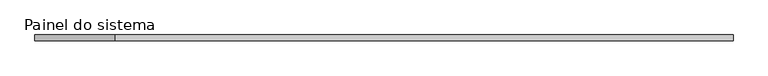
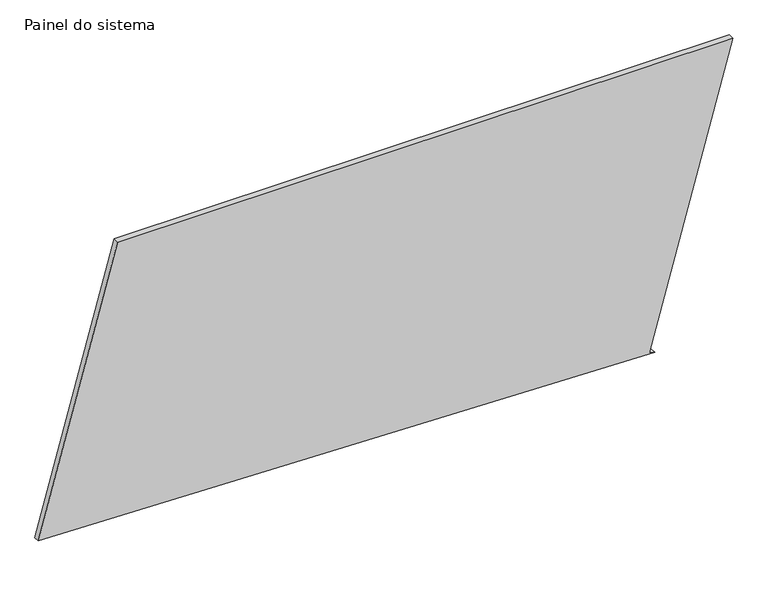
"""IFC4 building model written with IfcOpenShell, lengths in millimetres: plate geometry, Painel do sistema : Envidraçado."""

import ifcopenshell
import ifcopenshell.guid

model = None  # the IFC model being written
_history = None  # IfcOwnerHistory: only IFC2X3 demands one
_inside = {}  # id of a spatial element -> (the spatial element, [elements in it])
_under = {}  # id of a project, library or spatial element -> (it, [spatial elements below it])
_declared = {}  # id of a project -> (the project, [libraries it declares])
_typed = {}  # id of a type object -> (the type object, [elements of that type])
_made_of = {}  # id of a material, layer set ... -> (it, [elements and type objects made of it])


def new_model(schema):
    """Start an empty IFC model of exactly this schema.

    Asked for "IFC4X3", IfcOpenShell would pick the latest addendum, in which some entities
    have other attributes; the version numbers below select the first issue.
    IFC2X3 requires an IfcOwnerHistory on every rooted entity: one is made here for all.
    """
    global model, _history
    if schema == "IFC4X3":
        model = ifcopenshell.file(schema_version=(4, 3, 0, 0))
    else:
        model = ifcopenshell.file(schema=schema)
    _inside.clear()
    _under.clear()
    _declared.clear()
    _typed.clear()
    _made_of.clear()
    _history = None
    if model.schema == "IFC2X3":
        org = make("IfcOrganization", Name="unknown")
        user = make(
            "IfcPersonAndOrganization",
            ThePerson=make("IfcPerson", FamilyName="unknown"),
            TheOrganization=org,
        )
        app = make(
            "IfcApplication",
            ApplicationDeveloper=org,
            Version="unknown",
            ApplicationFullName="unknown",
            ApplicationIdentifier="unknown",
        )
        _history = make(
            "IfcOwnerHistory",
            OwningUser=user,
            OwningApplication=app,
            ChangeAction="ADDED",
            CreationDate=0,
        )
    return model


def make(cls, **values):
    """One entity of the class cls with the attributes given. An attribute that is None is left unset."""
    return model.create_entity(
        cls, **{name: value for name, value in values.items() if value is not None}
    )


def rooted(cls, **values):
    """An entity with a GlobalId (a new one), such as an element, a storey or a relation."""
    return make(cls, GlobalId=ifcopenshell.guid.new(), OwnerHistory=_history, **values)


def si_unit(unit_type, name, prefix=None):
    """IfcSIUnit, for example si_unit("LENGTHUNIT", "METRE", prefix="MILLI")."""
    return make("IfcSIUnit", UnitType=unit_type, Prefix=prefix, Name=name)


def assignment(units):
    """IfcUnitAssignment: the units of a project."""
    return None if units is None else make("IfcUnitAssignment", Units=units)


def point(xyz):
    """IfcCartesianPoint."""
    return None if xyz is None else make("IfcCartesianPoint", Coordinates=xyz)


def direction(xyz):
    """IfcDirection."""
    return None if xyz is None else make("IfcDirection", DirectionRatios=xyz)


def frame(location, z_axis=None, x_axis=None):
    """IfcAxis2Placement3D, a coordinate frame: its origin and axes. An axis left out is left unset."""
    return make(
        "IfcAxis2Placement3D",
        Location=point(location),
        Axis=direction(z_axis),
        RefDirection=direction(x_axis),
    )


def origin():
    """The frame at (0, 0, 0) with its axes left unset."""
    return frame((0.0, 0.0, 0.0))


def place(relative_to, where):
    """IfcLocalPlacement: puts the frame where relative to a parent placement (None: the world)."""
    return make(
        "IfcLocalPlacement", PlacementRelTo=relative_to, RelativePlacement=where
    )


def context(
    kind, dimensions, precision=None, world=None, true_north=None, identifier=None
):
    """IfcGeometricRepresentationContext, for example the 3D "Model" context."""
    return make(
        "IfcGeometricRepresentationContext",
        ContextIdentifier=identifier,
        ContextType=kind,
        CoordinateSpaceDimension=dimensions,
        Precision=precision,
        WorldCoordinateSystem=world,
        TrueNorth=true_north,
    )


def project(units=None, contexts=None):
    """IfcProject with its units and contexts."""
    return rooted(
        "IfcProject",
        Name="project",
        RepresentationContexts=contexts,
        UnitsInContext=assignment(units),
    )


def spatial(cls, under=None, at=None, **own):
    """A site, building, storey or space (cls), placed at a placement, below another one or the project."""
    s = rooted(cls, ObjectPlacement=at, **own)
    if under is not None:
        _under.setdefault(under.id(), (under, []))[1].append(s)
    return s


def polyline(points):
    """IfcPolyline through the points."""
    return make("IfcPolyline", Points=[point(p) for p in points])


def outline(outer, holes=None, kind="AREA"):
    """IfcArbitraryClosedProfileDef: a profile drawn as a closed curve; with holes, ...WithVoids."""
    if holes is None:
        return make("IfcArbitraryClosedProfileDef", ProfileType=kind, OuterCurve=outer)
    return make(
        "IfcArbitraryProfileDefWithVoids",
        ProfileType=kind,
        OuterCurve=outer,
        InnerCurves=holes,
    )


def extrude(swept, where, along, depth):
    """IfcExtrudedAreaSolid: the profile swept, set in the frame where, extruded along a direction by depth."""
    return make(
        "IfcExtrudedAreaSolid",
        SweptArea=swept,
        Position=where,
        ExtrudedDirection=direction(along),
        Depth=depth,
    )


def shape(context_of_items, identifier, shape_type, items):
    """IfcShapeRepresentation: the items that make up one representation, for example the "Body"."""
    return make(
        "IfcShapeRepresentation",
        ContextOfItems=context_of_items,
        RepresentationIdentifier=identifier,
        RepresentationType=shape_type,
        Items=items,
    )


def source(mapping_origin, context_of_items, identifier, shape_type, items):
    """IfcRepresentationMap: a shape defined once, which mapped items show again and again."""
    return make(
        "IfcRepresentationMap",
        MappingOrigin=mapping_origin,
        MappedRepresentation=shape(context_of_items, identifier, shape_type, items),
    )


def transform(
    local_origin,
    x_axis=None,
    y_axis=None,
    z_axis=None,
    scale=None,
    scale2=None,
    scale3=None,
    uniform=True,
):
    """IfcCartesianTransformationOperator3D, or its non-uniform kind. x_axis, y_axis, z_axis: its Axis1, 2, 3."""
    if uniform:
        return make(
            "IfcCartesianTransformationOperator3D",
            Axis1=direction(x_axis),
            Axis2=direction(y_axis),
            LocalOrigin=point(local_origin),
            Scale=scale,
            Axis3=direction(z_axis),
        )
    return make(
        "IfcCartesianTransformationOperator3DnonUniform",
        Axis1=direction(x_axis),
        Axis2=direction(y_axis),
        LocalOrigin=point(local_origin),
        Scale=scale,
        Axis3=direction(z_axis),
        Scale2=scale2,
        Scale3=scale3,
    )


def mapped(mapping_source, mapping_target):
    """IfcMappedItem: shows the shape of a source again, moved by a transform."""
    return make(
        "IfcMappedItem", MappingSource=mapping_source, MappingTarget=mapping_target
    )


def made_of(thing, what):
    """Note that an element or type object is made of a material, layer set ...; save() writes the relation."""
    if what is not None:
        _made_of.setdefault(what.id(), (what, []))[1].append(thing)
    return thing


def element(
    cls,
    number,
    at=None,
    inside=None,
    cuts=None,
    type_object=None,
    material=None,
    context=None,
    identifier="Body",
    shape_type=None,
    held_by="IfcProductDefinitionShape",
    body=None,
    shapes=None,
    **own,
):
    """One element of the class cls, such as IfcWall. Its Tag is "e" and its number.

    at: its placement. inside: the storey or other place that contains it. cuts: it is an
    opening in that element (IfcRelVoidsElement). A single representation is given by context,
    identifier, shape_type and body (its items); several are given by shapes. held_by: the class
    of the entity that holds the representations. save() writes the other relations.
    """
    e = rooted(cls, Tag="e%d" % number, ObjectPlacement=at, **own)
    if body is not None:
        shapes = [shape(context, identifier, shape_type, body)]
    if shapes is not None:
        e.Representation = make(held_by, Representations=shapes)
    if inside is not None:
        _inside.setdefault(inside.id(), (inside, []))[1].append(e)
    if cuts is not None:
        rooted(
            "IfcRelVoidsElement", RelatingBuildingElement=cuts, RelatedOpeningElement=e
        )
    if type_object is not None:
        _typed.setdefault(type_object.id(), (type_object, []))[1].append(e)
    return made_of(e, material)


def aggregate(whole, parts):
    """IfcRelAggregates: a whole, such as a stair, and the parts it consists of."""
    return rooted("IfcRelAggregates", RelatingObject=whole, RelatedObjects=parts)


def save(model, path):
    """Write the relations noted so far, then the file.

    IfcRelAggregates (storeys below a building ...), IfcRelContainedInSpatialStructure (elements
    in a storey), IfcRelDefinesByType, IfcRelAssociatesMaterial and IfcRelDeclares: one each for
    every whole, place, type object, material and project.
    """
    for whole, parts in _under.values():
        aggregate(whole, parts)
    for where, things in _inside.values():
        rooted(
            "IfcRelContainedInSpatialStructure",
            RelatedElements=things,
            RelatingStructure=where,
        )
    for kind, things in _typed.values():
        rooted("IfcRelDefinesByType", RelatedObjects=things, RelatingType=kind)
    for what, things in _made_of.values():
        rooted("IfcRelAssociatesMaterial", RelatedObjects=things, RelatingMaterial=what)
    for by, libraries in _declared.values():
        rooted("IfcRelDeclares", RelatingContext=by, RelatedDefinitions=libraries)
    model.write(path)


def painel_do_sistema_df5c15f3(model_context):
    return source(origin(), model_context, "Body", "SweptSolid", [
        extrude(outline(polyline([(0.0, 1157.1558687), (6.6310485, 1133.0513215), (1308.9960929, 1491.3258732), (1308.9960929, -1150.9442068), (71.6735371, -1491.3258732), (0.0, 1157.1558687)])), frame((0.0, 24.5, 0.0), z_axis=(0.0, 1.0, 0.0), x_axis=(0.0, 0.0, 1.0)), (0.0, 0.0, 1.0), 25.0),
    ])


if __name__ == "__main__":
    model = new_model("IFC4")
    model_context = context("Model", 3, world=origin())
    ifc_project = project(units=[si_unit("LENGTHUNIT", "METRE", prefix="MILLI")], contexts=[model_context])
    site = spatial("IfcSite", under=ifc_project)
    building = spatial("IfcBuilding", under=site)
    placement = place(None, origin())
    painel_do_sistema_shape = painel_do_sistema_df5c15f3(model_context)
    element("IfcPlate", 1, ObjectType="Painel do sistema : Envidraçado", at=placement, inside=building, context=model_context, shape_type="MappedRepresentation", body=[
        mapped(painel_do_sistema_shape, transform((0.0, 0.0, 0.0), x_axis=(1.0, 0.0, 0.0), y_axis=(0.0, 1.0, 0.0), z_axis=(0.0, 0.0, 1.0))),
    ])
    save(model, "model.ifc")

# Revit data of these elements
# Type "Painel do sistema : Envidraçado"
#   Construction Type Id = "GSP4R"
#   Analytic Construction = "Vidraça única Pilkington 1/8 pol"
#   Visual Light Transmittance = 0.9
#   Solar Heat Gain Coefficient = 0.86
#   Heat Transfer Coefficient (U) = 6.7069 W/(m²·K)
# Element 1 (IfcPlate, "Painel do sistema : Envidraçado")
#   Materials on its faces: "Vidro"
# Materials
#   "Vidro": class "Vidro", colour RGB 0 128 192, transparency 0.9, Description = "Vidro de sílica", Cost = 0
